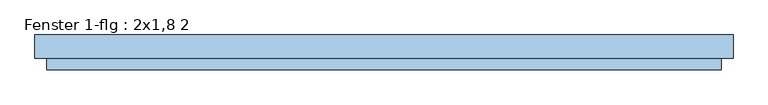
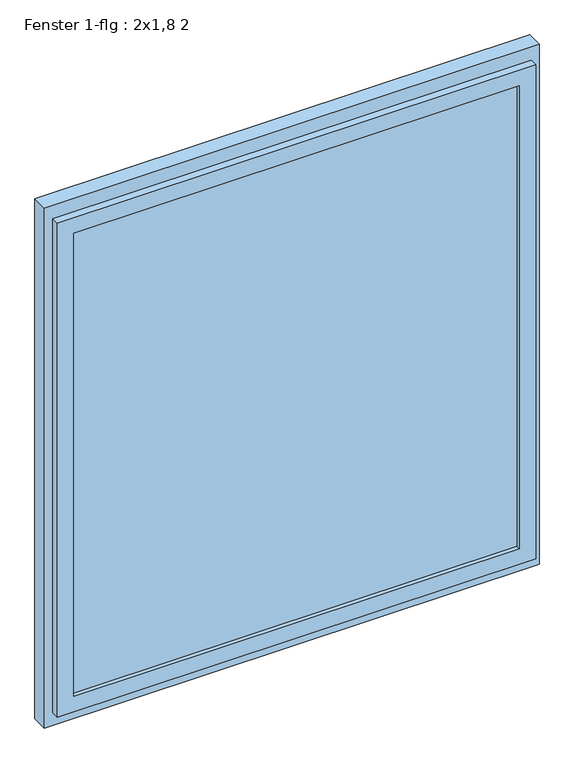
"""IFC4 building model written with IfcOpenShell, lengths in millimetres: window geometry, Fenster 1-flg : 2x1,8 2."""

import ifcopenshell
import ifcopenshell.guid

model = None  # the IFC model being written
_history = None  # IfcOwnerHistory: only IFC2X3 demands one
_inside = {}  # id of a spatial element -> (the spatial element, [elements in it])
_under = {}  # id of a project, library or spatial element -> (it, [spatial elements below it])
_declared = {}  # id of a project -> (the project, [libraries it declares])
_typed = {}  # id of a type object -> (the type object, [elements of that type])
_made_of = {}  # id of a material, layer set ... -> (it, [elements and type objects made of it])


def new_model(schema):
    """Start an empty IFC model of exactly this schema.

    Asked for "IFC4X3", IfcOpenShell would pick the latest addendum, in which some entities
    have other attributes; the version numbers below select the first issue.
    IFC2X3 requires an IfcOwnerHistory on every rooted entity: one is made here for all.
    """
    global model, _history
    if schema == "IFC4X3":
        model = ifcopenshell.file(schema_version=(4, 3, 0, 0))
    else:
        model = ifcopenshell.file(schema=schema)
    _inside.clear()
    _under.clear()
    _declared.clear()
    _typed.clear()
    _made_of.clear()
    _history = None
    if model.schema == "IFC2X3":
        org = make("IfcOrganization", Name="unknown")
        user = make(
            "IfcPersonAndOrganization",
            ThePerson=make("IfcPerson", FamilyName="unknown"),
            TheOrganization=org,
        )
        app = make(
            "IfcApplication",
            ApplicationDeveloper=org,
            Version="unknown",
            ApplicationFullName="unknown",
            ApplicationIdentifier="unknown",
        )
        _history = make(
            "IfcOwnerHistory",
            OwningUser=user,
            OwningApplication=app,
            ChangeAction="ADDED",
            CreationDate=0,
        )
    return model


def make(cls, **values):
    """One entity of the class cls with the attributes given. An attribute that is None is left unset."""
    return model.create_entity(
        cls, **{name: value for name, value in values.items() if value is not None}
    )


def rooted(cls, **values):
    """An entity with a GlobalId (a new one), such as an element, a storey or a relation."""
    return make(cls, GlobalId=ifcopenshell.guid.new(), OwnerHistory=_history, **values)


def si_unit(unit_type, name, prefix=None):
    """IfcSIUnit, for example si_unit("LENGTHUNIT", "METRE", prefix="MILLI")."""
    return make("IfcSIUnit", UnitType=unit_type, Prefix=prefix, Name=name)


def assignment(units):
    """IfcUnitAssignment: the units of a project."""
    return None if units is None else make("IfcUnitAssignment", Units=units)


def point(xyz):
    """IfcCartesianPoint."""
    return None if xyz is None else make("IfcCartesianPoint", Coordinates=xyz)


def direction(xyz):
    """IfcDirection."""
    return None if xyz is None else make("IfcDirection", DirectionRatios=xyz)


def frame(location, z_axis=None, x_axis=None):
    """IfcAxis2Placement3D, a coordinate frame: its origin and axes. An axis left out is left unset."""
    return make(
        "IfcAxis2Placement3D",
        Location=point(location),
        Axis=direction(z_axis),
        RefDirection=direction(x_axis),
    )


def origin():
    """The frame at (0, 0, 0) with its axes left unset."""
    return frame((0.0, 0.0, 0.0))


def place(relative_to, where):
    """IfcLocalPlacement: puts the frame where relative to a parent placement (None: the world)."""
    return make(
        "IfcLocalPlacement", PlacementRelTo=relative_to, RelativePlacement=where
    )


def context(
    kind, dimensions, precision=None, world=None, true_north=None, identifier=None
):
    """IfcGeometricRepresentationContext, for example the 3D "Model" context."""
    return make(
        "IfcGeometricRepresentationContext",
        ContextIdentifier=identifier,
        ContextType=kind,
        CoordinateSpaceDimension=dimensions,
        Precision=precision,
        WorldCoordinateSystem=world,
        TrueNorth=true_north,
    )


def project(units=None, contexts=None):
    """IfcProject with its units and contexts."""
    return rooted(
        "IfcProject",
        Name="project",
        RepresentationContexts=contexts,
        UnitsInContext=assignment(units),
    )


def spatial(cls, under=None, at=None, **own):
    """A site, building, storey or space (cls), placed at a placement, below another one or the project."""
    s = rooted(cls, ObjectPlacement=at, **own)
    if under is not None:
        _under.setdefault(under.id(), (under, []))[1].append(s)
    return s


def polyline(points):
    """IfcPolyline through the points."""
    return make("IfcPolyline", Points=[point(p) for p in points])


def outline(outer, holes=None, kind="AREA"):
    """IfcArbitraryClosedProfileDef: a profile drawn as a closed curve; with holes, ...WithVoids."""
    if holes is None:
        return make("IfcArbitraryClosedProfileDef", ProfileType=kind, OuterCurve=outer)
    return make(
        "IfcArbitraryProfileDefWithVoids",
        ProfileType=kind,
        OuterCurve=outer,
        InnerCurves=holes,
    )


def extrude(swept, where, along, depth):
    """IfcExtrudedAreaSolid: the profile swept, set in the frame where, extruded along a direction by depth."""
    return make(
        "IfcExtrudedAreaSolid",
        SweptArea=swept,
        Position=where,
        ExtrudedDirection=direction(along),
        Depth=depth,
    )


def faces_of(points, faces, orient=None, outer=None):
    """IfcFace entities. A face is a list of loops; a loop is a list of indices into points, from 0.

    orient and outer hold one flag for each loop. By default every Orientation is true, the
    first loop of a face is its IfcFaceOuterBound and the others are IfcFaceBound.
    """
    made = []
    for i, loops in enumerate(faces):
        bounds = []
        for j, loop in enumerate(loops):
            is_outer = j == 0 if outer is None else outer[i][j]
            bounds.append(
                make(
                    "IfcFaceOuterBound" if is_outer else "IfcFaceBound",
                    Bound=make("IfcPolyLoop", Polygon=[points[k] for k in loop]),
                    Orientation=True if orient is None else orient[i][j],
                )
            )
        made.append(make("IfcFace", Bounds=bounds))
    return made


def faceted_brep(points, faces, orient=None, outer=None, voids=None):
    """IfcFacetedBrep: a solid bounded by flat faces; with voids (closed shells), ...WithVoids."""
    shared = [point(p) for p in points]
    hull = make("IfcClosedShell", CfsFaces=faces_of(shared, faces, orient, outer))
    if voids is None:
        return make("IfcFacetedBrep", Outer=hull)
    return make(
        "IfcFacetedBrepWithVoids",
        Outer=hull,
        Voids=[
            make(cls, CfsFaces=faces_of(shared, fs, o, b)) for cls, fs, o, b in voids
        ],
    )


def shape(context_of_items, identifier, shape_type, items):
    """IfcShapeRepresentation: the items that make up one representation, for example the "Body"."""
    return make(
        "IfcShapeRepresentation",
        ContextOfItems=context_of_items,
        RepresentationIdentifier=identifier,
        RepresentationType=shape_type,
        Items=items,
    )


def source(mapping_origin, context_of_items, identifier, shape_type, items):
    """IfcRepresentationMap: a shape defined once, which mapped items show again and again."""
    return make(
        "IfcRepresentationMap",
        MappingOrigin=mapping_origin,
        MappedRepresentation=shape(context_of_items, identifier, shape_type, items),
    )


def transform(
    local_origin,
    x_axis=None,
    y_axis=None,
    z_axis=None,
    scale=None,
    scale2=None,
    scale3=None,
    uniform=True,
):
    """IfcCartesianTransformationOperator3D, or its non-uniform kind. x_axis, y_axis, z_axis: its Axis1, 2, 3."""
    if uniform:
        return make(
            "IfcCartesianTransformationOperator3D",
            Axis1=direction(x_axis),
            Axis2=direction(y_axis),
            LocalOrigin=point(local_origin),
            Scale=scale,
            Axis3=direction(z_axis),
        )
    return make(
        "IfcCartesianTransformationOperator3DnonUniform",
        Axis1=direction(x_axis),
        Axis2=direction(y_axis),
        LocalOrigin=point(local_origin),
        Scale=scale,
        Axis3=direction(z_axis),
        Scale2=scale2,
        Scale3=scale3,
    )


def mapped(mapping_source, mapping_target):
    """IfcMappedItem: shows the shape of a source again, moved by a transform."""
    return make(
        "IfcMappedItem", MappingSource=mapping_source, MappingTarget=mapping_target
    )


def made_of(thing, what):
    """Note that an element or type object is made of a material, layer set ...; save() writes the relation."""
    if what is not None:
        _made_of.setdefault(what.id(), (what, []))[1].append(thing)
    return thing


def element(
    cls,
    number,
    at=None,
    inside=None,
    cuts=None,
    type_object=None,
    material=None,
    context=None,
    identifier="Body",
    shape_type=None,
    held_by="IfcProductDefinitionShape",
    body=None,
    shapes=None,
    **own,
):
    """One element of the class cls, such as IfcWall. Its Tag is "e" and its number.

    at: its placement. inside: the storey or other place that contains it. cuts: it is an
    opening in that element (IfcRelVoidsElement). A single representation is given by context,
    identifier, shape_type and body (its items); several are given by shapes. held_by: the class
    of the entity that holds the representations. save() writes the other relations.
    """
    e = rooted(cls, Tag="e%d" % number, ObjectPlacement=at, **own)
    if body is not None:
        shapes = [shape(context, identifier, shape_type, body)]
    if shapes is not None:
        e.Representation = make(held_by, Representations=shapes)
    if inside is not None:
        _inside.setdefault(inside.id(), (inside, []))[1].append(e)
    if cuts is not None:
        rooted(
            "IfcRelVoidsElement", RelatingBuildingElement=cuts, RelatedOpeningElement=e
        )
    if type_object is not None:
        _typed.setdefault(type_object.id(), (type_object, []))[1].append(e)
    return made_of(e, material)


def aggregate(whole, parts):
    """IfcRelAggregates: a whole, such as a stair, and the parts it consists of."""
    return rooted("IfcRelAggregates", RelatingObject=whole, RelatedObjects=parts)


def save(model, path):
    """Write the relations noted so far, then the file.

    IfcRelAggregates (storeys below a building ...), IfcRelContainedInSpatialStructure (elements
    in a storey), IfcRelDefinesByType, IfcRelAssociatesMaterial and IfcRelDeclares: one each for
    every whole, place, type object, material and project.
    """
    for whole, parts in _under.values():
        aggregate(whole, parts)
    for where, things in _inside.values():
        rooted(
            "IfcRelContainedInSpatialStructure",
            RelatedElements=things,
            RelatingStructure=where,
        )
    for kind, things in _typed.values():
        rooted("IfcRelDefinesByType", RelatedObjects=things, RelatingType=kind)
    for what, things in _made_of.values():
        rooted("IfcRelAssociatesMaterial", RelatedObjects=things, RelatingMaterial=what)
    for by, libraries in _declared.values():
        rooted("IfcRelDeclares", RelatingContext=by, RelatedDefinitions=libraries)
    model.write(path)


def fenster_1_flg_2x1_8_2_041d18e4(model_context):
    return source(origin(), model_context, "Body", "SolidModel", [
        extrude(outline(polyline([(3000.0, 900.0), (3000.0, -900.0), (1000.0, -900.0), (1000.0, 900.0), (3000.0, 900.0)]), holes=[polyline([(2920.0, 840.0), (1080.0, 840.0), (1080.0, -840.0), (2920.0, -840.0), (2920.0, 840.0)])]), frame((0.0, 20.0, 0.0), z_axis=(0.0, 1.0, 0.0), x_axis=(0.0, 0.0, 1.0)), (0.0, 0.0, 1.0), 60.0),
        faceted_brep([(870.0, 20.0, 2950.0), (870.0, -10.0, 2950.0), (870.0, -10.0, 1050.0), (870.0, 20.0, 1050.0), (-870.0, -10.0, 2950.0), (-870.0, -10.0, 1050.0), (810.0, -10.0, 1110.0), (-810.0, -10.0, 1110.0), (-810.0, -10.0, 2890.0), (810.0, -10.0, 2890.0), (-870.0, 20.0, 1050.0), (-870.0, 20.0, 2950.0), (840.0, 20.0, 2920.0), (-840.0, 20.0, 2920.0), (-840.0, 20.0, 1080.0), (840.0, 20.0, 1080.0), (840.0, 50.0, 2920.0), (840.0, 50.0, 1080.0), (-840.0, 50.0, 1080.0), (-840.0, 50.0, 2920.0), (810.0, 50.0, 2890.0), (-810.0, 50.0, 2890.0), (-810.0, 50.0, 1110.0), (810.0, 50.0, 1110.0)], [[[0, 1, 2, 3]], [[1, 4, 5, 2], [6, 7, 8, 9]], [[3, 2, 5, 10]], [[3, 10, 11, 0], [12, 13, 14, 15]], [[16, 12, 15, 17]], [[17, 15, 14, 18]], [[17, 18, 19, 16], [20, 21, 22, 23]], [[9, 20, 23, 6]], [[6, 23, 22, 7]], [[10, 5, 4, 11]], [[18, 14, 13, 19]], [[7, 22, 21, 8]], [[11, 4, 1, 0]], [[19, 13, 12, 16]], [[8, 21, 20, 9]]]),
        extrude(outline(polyline([(810.0, 5.0), (-810.0, 5.0), (-810.0, 35.0), (810.0, 35.0), (810.0, 5.0)])), frame((0.0, 0.0, 1110.0), z_axis=(0.0, 0.0, 1.0), x_axis=(1.0, 0.0, 0.0)), (0.0, 0.0, 1.0), 1780.0),
    ])


if __name__ == "__main__":
    model = new_model("IFC4")
    model_context = context("Model", 3, world=origin())
    ifc_project = project(units=[si_unit("LENGTHUNIT", "METRE", prefix="MILLI")], contexts=[model_context])
    site = spatial("IfcSite", under=ifc_project)
    building = spatial("IfcBuilding", under=site)
    placement = place(None, origin())
    fenster_1_flg_2x1_8_2_shape = fenster_1_flg_2x1_8_2_041d18e4(model_context)
    element("IfcWindow", 1, ObjectType="Fenster 1-flg : 2x1,8 2", at=placement, inside=building, context=model_context, shape_type="MappedRepresentation", body=[
        mapped(fenster_1_flg_2x1_8_2_shape, transform((0.0, 0.0, 0.0), x_axis=(1.0, 0.0, 0.0), y_axis=(0.0, 1.0, 0.0), z_axis=(0.0, 0.0, 1.0))),
    ])
    save(model, "model.ifc")

# Revit data of these elements
# Type "Fenster 1-flg : 2x1,8 2"
#   Type Mark = "69"
#   Operation = "SinglePanel"
#   Keynote = "16.05.01"
#   Visual Light Transmittance = 0.9
#   Solar Heat Gain Coefficient = 0.86
#   Rough Width = 1.800 m
#   Rough Height = 2.000 m
#   Heat Transfer Coefficient (U) = 5.5617 W/(m²·K)
#   Rahmentiefe = 0.060 m
#   Rahmenhöhe - unten = 0.080 m
#   Rahmenhöhe - oben = 0.080 m
#   Rahmenbreite = 0.060 m
#   Height = 2.000 m
#   Tiefe Flügel = 0.060 m
#   Flügelbreite = 0.060 m
#   Einbautiefe (von außen) [instance default] = 0.100 m
#   Width = 1.800 m
#   Klappflügel [instance default] = no
#   Kippflügel [instance default] = yes
#   Öffnungsrichtung in Draufsicht anzeigen [instance default] = no
#   Drehflügel 1 [instance default] = yes
#   Rahmen 1 [instance default] = none
#   Glas [instance default] = none
#   Flügel [instance default] = none
#   Fensterbank Innenseite [instance default] = none
#   Fensterbank Außenseite [instance default] = none
#   Construction Type Id = ""
#   Wall Closure = (empty or 0)
#   Analytic Construction = (empty or 0)
# Element 1 (IfcWindow, "Fenster 1-flg : 2x1,8 2")
#   Einbautiefe (von außen) = 0.230 m
#   Materials on its faces: "Kunststoff - Weiß", "Glas"
# Materials
#   "Kunststoff - Weiß": class "Kunststoff", colour RGB 249 249 249, transparency 0, Cost = 0
#   "Glas": class "Glas", colour RGB 0 0 255, transparency 0.75, Comments = "Render-Darstellung nicht aktualisiert ", Cost = 0
